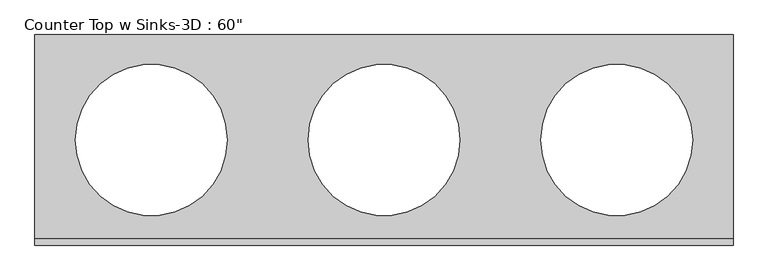
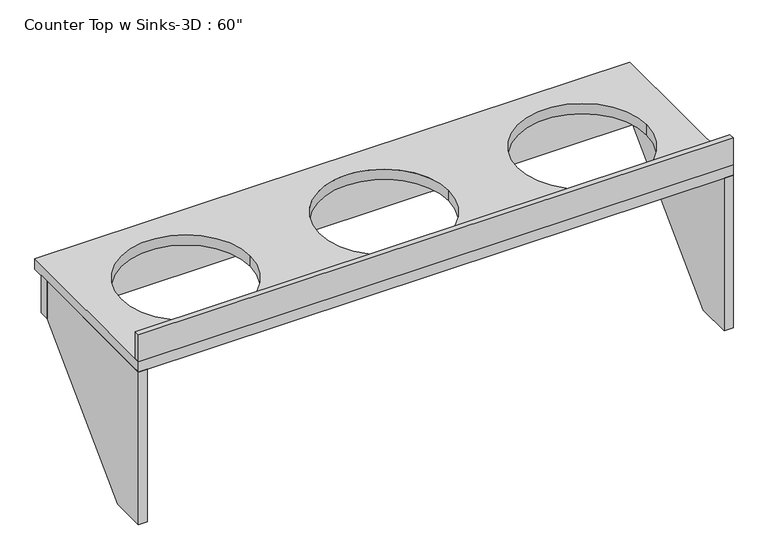
"""IFC4 building model written with IfcOpenShell, lengths in millimetres: furniture geometry."""

from ifc_helpers import new_model, si_unit, point, frame, frame_2d, origin, place, context, project, spatial, polyline, circle_curve, trimmed, segment, composite_curve, outline, extrude, source, transform, mapped, element, save


def furniture_935aa8e9(model_context):
    return source(origin(), model_context, "Body", "SweptSolid", [
        extrude(outline(polyline([(198.4375, 825.5), (757.2375, 825.5), (757.2375, 685.8), (325.4375, 254.0), (198.4375, 254.0), (198.4375, 825.5)])), frame((-1116.1103038, 0.0, 0.0), z_axis=(1.0, 0.0, 0.0), x_axis=(0.0, 1.0, 0.0)), (0.0, 0.0, 1.0), 31.75),
        extrude(outline(polyline([(198.4375, 825.5), (757.2375, 825.5), (757.2375, 685.8), (325.4375, 254.0), (198.4375, 254.0), (198.4375, 825.5)])), frame((957.1646962, 0.0, 0.0), z_axis=(1.0, 0.0, 0.0), x_axis=(0.0, 1.0, 0.0)), (0.0, 0.0, 1.0), 31.75),
        extrude(outline(polyline([(-1116.1103038, 757.2375), (-1116.1103038, 795.3375), (988.9146962, 795.3375), (988.9146962, 757.2375), (-1116.1103038, 757.2375)])), frame((0.0, 0.0, 685.8), z_axis=(0.0, 0.0, 1.0), x_axis=(1.0, 0.0, 0.0)), (0.0, 0.0, 1.0), 139.7),
        extrude(outline(polyline([(988.9146962, 198.4375), (-1116.1103038, 198.4375), (-1116.1103038, 217.4875), (988.9146962, 217.4875), (988.9146962, 198.4375)])), frame((0.0, 0.0, 863.6), z_axis=(0.0, 0.0, 1.0), x_axis=(1.0, 0.0, 0.0)), (0.0, 0.0, 1.0), 101.6),
        extrude(outline(polyline([(988.9146962, 198.4375), (-1116.1103038, 198.4375), (-1116.1103038, 833.4375), (988.9146962, 833.4375), (988.9146962, 198.4375)]), holes=[composite_curve([segment(trimmed(circle_curve(frame_2d((-765.2728038, 515.9375)), 228.6), [point((-993.8728038, 515.9375))], [point((-536.6728038, 515.9375))], True, "CARTESIAN"), True, "CONTINUOUS"), segment(trimmed(circle_curve(frame_2d((-765.2728038, 515.9375)), 228.6), [point((-536.6728038, 515.9375))], [point((-993.8728038, 515.9375))], True, "CARTESIAN"), True, "CONTINUOUS")], self_intersect=False), composite_curve([segment(trimmed(circle_curve(frame_2d((638.0771962, 515.9375)), 228.6), [point((409.4771962, 515.9375))], [point((866.6771962, 515.9375))], True, "CARTESIAN"), True, "CONTINUOUS"), segment(trimmed(circle_curve(frame_2d((638.0771962, 515.9375)), 228.6), [point((866.6771962, 515.9375))], [point((409.4771962, 515.9375))], True, "CARTESIAN"), True, "CONTINUOUS")], self_intersect=False), composite_curve([segment(trimmed(circle_curve(frame_2d((-63.5978038, 515.9375)), 228.6), [point((-292.1978038, 515.9375))], [point((165.0021962, 515.9375))], True, "CARTESIAN"), True, "CONTINUOUS"), segment(trimmed(circle_curve(frame_2d((-63.5978038, 515.9375)), 228.6), [point((165.0021962, 515.9375))], [point((-292.1978038, 515.9375))], True, "CARTESIAN"), True, "CONTINUOUS")], self_intersect=False)]), frame((0.0, 0.0, 825.5), z_axis=(0.0, 0.0, 1.0), x_axis=(1.0, 0.0, 0.0)), (0.0, 0.0, 1.0), 38.1),
    ])


if __name__ == "__main__":
    model = new_model("IFC4")
    model_context = context("Model", 3, world=origin())
    ifc_project = project(units=[si_unit("LENGTHUNIT", "METRE", prefix="MILLI")], contexts=[model_context])
    site = spatial("IfcSite", under=ifc_project)
    building = spatial("IfcBuilding", under=site)
    placement = place(None, origin())
    furniture_shape = furniture_935aa8e9(model_context)
    element("IfcFurniture", 1, ObjectType="Counter Top w Sinks-3D : 60\"", at=placement, inside=building, context=model_context, shape_type="MappedRepresentation", body=[
        mapped(furniture_shape, transform((0.0, 0.0, 0.0), x_axis=(1.0, 0.0, 0.0), y_axis=(0.0, 1.0, 0.0), z_axis=(0.0, 0.0, 1.0))),
    ])
    save(model, "model.ifc")

# Revit data of these elements
# Type "Counter Top w Sinks-3D : 60\""
#   Assembly Code = "C1030400"
#   Height = 2' - 10"
#   Distance To Sink Center [instance default] = 1' - 3"
#   Clear Space = 2' - 3"
#   Counter Thickness = 0' - 1 1/2"
#   Depth = 2' - 1"
#   Length [instance default] = 5' - 0"
#   Number Of Sinks [instance default] = 2
#   Counter Top Material = Counter Top
#   Base Material = Laminate
#   Default Elevation = 0
# Element 1 (IfcFurniture, "Counter Top w Sinks-3D : 60\"")
#   Distance To Sink Center = 1' - 1 13/16"
#   Length = 6' - 10 7/8"
#   Number Of Sinks = 3
#   Materials on its faces: "Counter Top", "Laminate"
# Materials
#   "Counter Top": class "Unassigned", colour RGB 247 247 239, transparency 0
#   "Laminate": class "Unassigned", colour RGB 247 235 201, transparency 0
